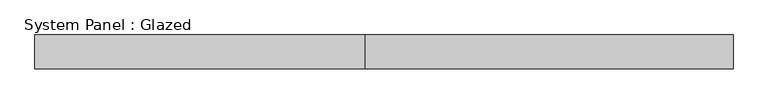
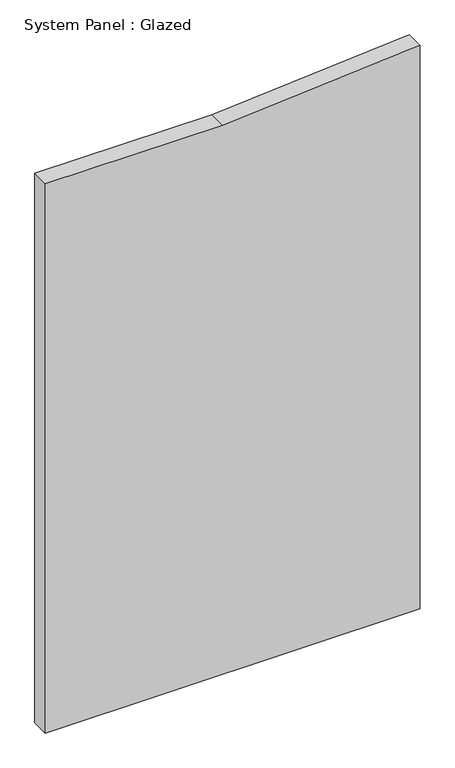
"""IFC4 building model written with IfcOpenShell, lengths in millimetres: plate geometry, System Panel : Glazed."""

from ifc_helpers import new_model, si_unit, frame, origin, place, context, project, spatial, polyline, outline, extrude, source, transform, mapped, element, save


def system_panel_glazed_d6fbae79(model_context):
    return source(origin(), model_context, "Body", "SweptSolid", [
        extrude(outline(polyline([(0.0, -519.5), (0.0, 519.5), (1651.9724847, 519.5), (1610.0, -28.1808092), (1610.0, -519.5), (0.0, -519.5)])), frame((0.0, -25.0, 0.0), z_axis=(0.0, 1.0, 0.0), x_axis=(0.0, 0.0, 1.0)), (0.0, 0.0, 1.0), 50.0),
    ])


if __name__ == "__main__":
    model = new_model("IFC4")
    model_context = context("Model", 3, world=origin())
    ifc_project = project(units=[si_unit("LENGTHUNIT", "METRE", prefix="MILLI")], contexts=[model_context])
    site = spatial("IfcSite", under=ifc_project)
    building = spatial("IfcBuilding", under=site)
    placement = place(None, origin())
    system_panel_glazed_shape = system_panel_glazed_d6fbae79(model_context)
    element("IfcPlate", 1, ObjectType="System Panel : Glazed", at=placement, inside=building, context=model_context, shape_type="MappedRepresentation", body=[
        mapped(system_panel_glazed_shape, transform((0.0, 0.0, 0.0), x_axis=(1.0, 0.0, 0.0), y_axis=(0.0, 1.0, 0.0), z_axis=(0.0, 0.0, 1.0))),
    ])
    save(model, "model.ifc")

# Revit data of these elements
# Type "System Panel : Glazed"
#   Type Mark = "CW-GLASS"
# Element 1 (IfcPlate, "System Panel : Glazed")
#   Materials on its faces: "Glass_Clear"
# Materials
#   "Glass_Clear": class "Glass", colour RGB 128 128 255, transparency 0.8, Comments = "Rendering appearance not upgraded ", Cost = 0
